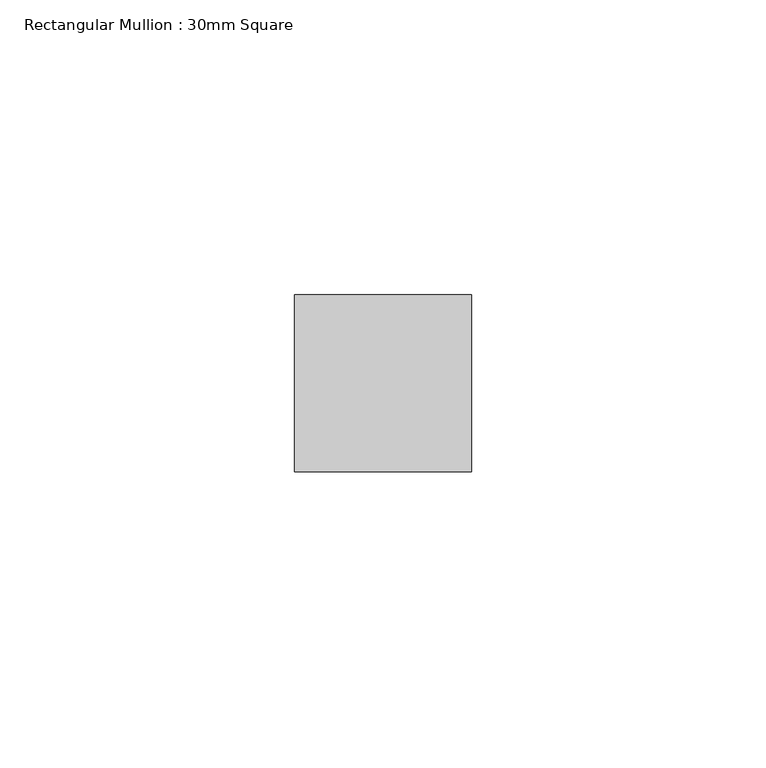
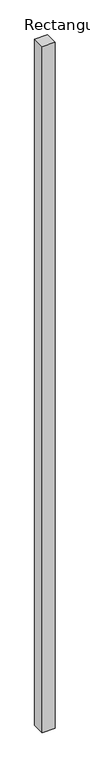
"""IFC4 building model written with IfcOpenShell, lengths in millimetres: member geometry, Rectangular Mullion : 30mm Square."""

from ifc_helpers import new_model, si_unit, frame, origin, place, context, project, spatial, polyline, outline, extrude, source, transform, mapped, element, save


def rectangular_mullion_30mm_square_06158fc0(model_context):
    return source(origin(), model_context, "Body", "SweptSolid", [
        extrude(outline(polyline([(15.0, 15.0), (15.0, -15.0), (-15.0, -15.0), (-15.0, 15.0), (15.0, 15.0)])), frame((0.0, 0.0, -1668.6160358), z_axis=(0.0, 0.0, 1.0), x_axis=(1.0, 0.0, 0.0)), (0.0, 0.0, 1.0), 1668.6160358),
    ])


if __name__ == "__main__":
    model = new_model("IFC4")
    model_context = context("Model", 3, world=origin())
    ifc_project = project(units=[si_unit("LENGTHUNIT", "METRE", prefix="MILLI")], contexts=[model_context])
    site = spatial("IfcSite", under=ifc_project)
    building = spatial("IfcBuilding", under=site)
    placement = place(None, origin())
    rectangular_mullion_30mm_square_shape = rectangular_mullion_30mm_square_06158fc0(model_context)
    element("IfcMember", 1, ObjectType="Rectangular Mullion : 30mm Square", at=placement, inside=building, context=model_context, shape_type="MappedRepresentation", body=[
        mapped(rectangular_mullion_30mm_square_shape, transform((0.0, 0.0, 0.0), x_axis=(1.0, 0.0, 0.0), y_axis=(0.0, 1.0, 0.0), z_axis=(0.0, 0.0, 1.0))),
    ])
    save(model, "model.ifc")

# Revit data of these elements
# Type "Rectangular Mullion : 30mm Square"
#   built-in parameter 1007304 = 0.0984252 (stored number, unit not read)
#   built-in parameter 1007301 = 0.0492126 (stored number, unit not read)
#   built-in parameter 1007300 = 0.0492126 (stored number, unit not read)
# Element 1 (IfcMember, "Rectangular Mullion : 30mm Square")
#   Materials on its faces: "Aluminum"
# Materials
#   "Aluminum": class "Metal", colour RGB 244 244 244, transparency 0, Description = "Aluminum 6061", Cost = 0
